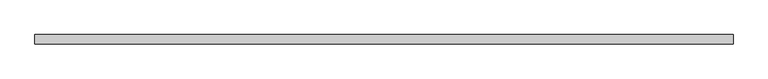
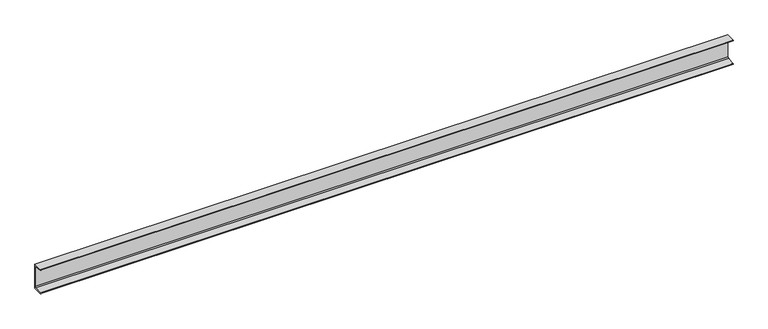
"""IFC4 building model written with IfcOpenShell, lengths in millimetres: beam geometry, C-образный профиль (ГОСТ 8240-89) Балки : [ 22."""

import ifcopenshell
import ifcopenshell.guid

model = None  # the IFC model being written
_history = None  # IfcOwnerHistory: only IFC2X3 demands one
_inside = {}  # id of a spatial element -> (the spatial element, [elements in it])
_under = {}  # id of a project, library or spatial element -> (it, [spatial elements below it])
_declared = {}  # id of a project -> (the project, [libraries it declares])
_typed = {}  # id of a type object -> (the type object, [elements of that type])
_made_of = {}  # id of a material, layer set ... -> (it, [elements and type objects made of it])


def new_model(schema):
    """Start an empty IFC model of exactly this schema.

    Asked for "IFC4X3", IfcOpenShell would pick the latest addendum, in which some entities
    have other attributes; the version numbers below select the first issue.
    IFC2X3 requires an IfcOwnerHistory on every rooted entity: one is made here for all.
    """
    global model, _history
    if schema == "IFC4X3":
        model = ifcopenshell.file(schema_version=(4, 3, 0, 0))
    else:
        model = ifcopenshell.file(schema=schema)
    _inside.clear()
    _under.clear()
    _declared.clear()
    _typed.clear()
    _made_of.clear()
    _history = None
    if model.schema == "IFC2X3":
        org = make("IfcOrganization", Name="unknown")
        user = make(
            "IfcPersonAndOrganization",
            ThePerson=make("IfcPerson", FamilyName="unknown"),
            TheOrganization=org,
        )
        app = make(
            "IfcApplication",
            ApplicationDeveloper=org,
            Version="unknown",
            ApplicationFullName="unknown",
            ApplicationIdentifier="unknown",
        )
        _history = make(
            "IfcOwnerHistory",
            OwningUser=user,
            OwningApplication=app,
            ChangeAction="ADDED",
            CreationDate=0,
        )
    return model


def make(cls, **values):
    """One entity of the class cls with the attributes given. An attribute that is None is left unset."""
    return model.create_entity(
        cls, **{name: value for name, value in values.items() if value is not None}
    )


def rooted(cls, **values):
    """An entity with a GlobalId (a new one), such as an element, a storey or a relation."""
    return make(cls, GlobalId=ifcopenshell.guid.new(), OwnerHistory=_history, **values)


def si_unit(unit_type, name, prefix=None):
    """IfcSIUnit, for example si_unit("LENGTHUNIT", "METRE", prefix="MILLI")."""
    return make("IfcSIUnit", UnitType=unit_type, Prefix=prefix, Name=name)


def assignment(units):
    """IfcUnitAssignment: the units of a project."""
    return None if units is None else make("IfcUnitAssignment", Units=units)


def point(xyz):
    """IfcCartesianPoint."""
    return None if xyz is None else make("IfcCartesianPoint", Coordinates=xyz)


def direction(xyz):
    """IfcDirection."""
    return None if xyz is None else make("IfcDirection", DirectionRatios=xyz)


def frame(location, z_axis=None, x_axis=None):
    """IfcAxis2Placement3D, a coordinate frame: its origin and axes. An axis left out is left unset."""
    return make(
        "IfcAxis2Placement3D",
        Location=point(location),
        Axis=direction(z_axis),
        RefDirection=direction(x_axis),
    )


def frame_2d(location, x_axis=None):
    """IfcAxis2Placement2D, a coordinate frame in the plane: its origin and x axis."""
    return make(
        "IfcAxis2Placement2D", Location=point(location), RefDirection=direction(x_axis)
    )


def origin():
    """The frame at (0, 0, 0) with its axes left unset."""
    return frame((0.0, 0.0, 0.0))


def place(relative_to, where):
    """IfcLocalPlacement: puts the frame where relative to a parent placement (None: the world)."""
    return make(
        "IfcLocalPlacement", PlacementRelTo=relative_to, RelativePlacement=where
    )


def context(
    kind, dimensions, precision=None, world=None, true_north=None, identifier=None
):
    """IfcGeometricRepresentationContext, for example the 3D "Model" context."""
    return make(
        "IfcGeometricRepresentationContext",
        ContextIdentifier=identifier,
        ContextType=kind,
        CoordinateSpaceDimension=dimensions,
        Precision=precision,
        WorldCoordinateSystem=world,
        TrueNorth=true_north,
    )


def project(units=None, contexts=None):
    """IfcProject with its units and contexts."""
    return rooted(
        "IfcProject",
        Name="project",
        RepresentationContexts=contexts,
        UnitsInContext=assignment(units),
    )


def spatial(cls, under=None, at=None, **own):
    """A site, building, storey or space (cls), placed at a placement, below another one or the project."""
    s = rooted(cls, ObjectPlacement=at, **own)
    if under is not None:
        _under.setdefault(under.id(), (under, []))[1].append(s)
    return s


def polyline(points):
    """IfcPolyline through the points."""
    return make("IfcPolyline", Points=[point(p) for p in points])


def circle_curve(where, radius):
    """IfcCircle in the frame where."""
    return make("IfcCircle", Position=where, Radius=radius)


def trimmed(basis, trim1, trim2, sense, master):
    """IfcTrimmedCurve: the piece of a basis curve between two trims."""
    return make(
        "IfcTrimmedCurve",
        BasisCurve=basis,
        Trim1=trim1,
        Trim2=trim2,
        SenseAgreement=sense,
        MasterRepresentation=master,
    )


def segment(curve, same_sense, transition):
    """IfcCompositeCurveSegment."""
    return make(
        "IfcCompositeCurveSegment",
        Transition=transition,
        SameSense=same_sense,
        ParentCurve=curve,
    )


def composite_curve(segments, self_intersect=None):
    """IfcCompositeCurve: segments joined end to end."""
    return make("IfcCompositeCurve", Segments=segments, SelfIntersect=self_intersect)


def outline(outer, holes=None, kind="AREA"):
    """IfcArbitraryClosedProfileDef: a profile drawn as a closed curve; with holes, ...WithVoids."""
    if holes is None:
        return make("IfcArbitraryClosedProfileDef", ProfileType=kind, OuterCurve=outer)
    return make(
        "IfcArbitraryProfileDefWithVoids",
        ProfileType=kind,
        OuterCurve=outer,
        InnerCurves=holes,
    )


def extrude(swept, where, along, depth):
    """IfcExtrudedAreaSolid: the profile swept, set in the frame where, extruded along a direction by depth."""
    return make(
        "IfcExtrudedAreaSolid",
        SweptArea=swept,
        Position=where,
        ExtrudedDirection=direction(along),
        Depth=depth,
    )


def shape(context_of_items, identifier, shape_type, items):
    """IfcShapeRepresentation: the items that make up one representation, for example the "Body"."""
    return make(
        "IfcShapeRepresentation",
        ContextOfItems=context_of_items,
        RepresentationIdentifier=identifier,
        RepresentationType=shape_type,
        Items=items,
    )


def source(mapping_origin, context_of_items, identifier, shape_type, items):
    """IfcRepresentationMap: a shape defined once, which mapped items show again and again."""
    return make(
        "IfcRepresentationMap",
        MappingOrigin=mapping_origin,
        MappedRepresentation=shape(context_of_items, identifier, shape_type, items),
    )


def transform(
    local_origin,
    x_axis=None,
    y_axis=None,
    z_axis=None,
    scale=None,
    scale2=None,
    scale3=None,
    uniform=True,
):
    """IfcCartesianTransformationOperator3D, or its non-uniform kind. x_axis, y_axis, z_axis: its Axis1, 2, 3."""
    if uniform:
        return make(
            "IfcCartesianTransformationOperator3D",
            Axis1=direction(x_axis),
            Axis2=direction(y_axis),
            LocalOrigin=point(local_origin),
            Scale=scale,
            Axis3=direction(z_axis),
        )
    return make(
        "IfcCartesianTransformationOperator3DnonUniform",
        Axis1=direction(x_axis),
        Axis2=direction(y_axis),
        LocalOrigin=point(local_origin),
        Scale=scale,
        Axis3=direction(z_axis),
        Scale2=scale2,
        Scale3=scale3,
    )


def mapped(mapping_source, mapping_target):
    """IfcMappedItem: shows the shape of a source again, moved by a transform."""
    return make(
        "IfcMappedItem", MappingSource=mapping_source, MappingTarget=mapping_target
    )


def made_of(thing, what):
    """Note that an element or type object is made of a material, layer set ...; save() writes the relation."""
    if what is not None:
        _made_of.setdefault(what.id(), (what, []))[1].append(thing)
    return thing


def element(
    cls,
    number,
    at=None,
    inside=None,
    cuts=None,
    type_object=None,
    material=None,
    context=None,
    identifier="Body",
    shape_type=None,
    held_by="IfcProductDefinitionShape",
    body=None,
    shapes=None,
    **own,
):
    """One element of the class cls, such as IfcWall. Its Tag is "e" and its number.

    at: its placement. inside: the storey or other place that contains it. cuts: it is an
    opening in that element (IfcRelVoidsElement). A single representation is given by context,
    identifier, shape_type and body (its items); several are given by shapes. held_by: the class
    of the entity that holds the representations. save() writes the other relations.
    """
    e = rooted(cls, Tag="e%d" % number, ObjectPlacement=at, **own)
    if body is not None:
        shapes = [shape(context, identifier, shape_type, body)]
    if shapes is not None:
        e.Representation = make(held_by, Representations=shapes)
    if inside is not None:
        _inside.setdefault(inside.id(), (inside, []))[1].append(e)
    if cuts is not None:
        rooted(
            "IfcRelVoidsElement", RelatingBuildingElement=cuts, RelatedOpeningElement=e
        )
    if type_object is not None:
        _typed.setdefault(type_object.id(), (type_object, []))[1].append(e)
    return made_of(e, material)


def aggregate(whole, parts):
    """IfcRelAggregates: a whole, such as a stair, and the parts it consists of."""
    return rooted("IfcRelAggregates", RelatingObject=whole, RelatedObjects=parts)


def save(model, path):
    """Write the relations noted so far, then the file.

    IfcRelAggregates (storeys below a building ...), IfcRelContainedInSpatialStructure (elements
    in a storey), IfcRelDefinesByType, IfcRelAssociatesMaterial and IfcRelDeclares: one each for
    every whole, place, type object, material and project.
    """
    for whole, parts in _under.values():
        aggregate(whole, parts)
    for where, things in _inside.values():
        rooted(
            "IfcRelContainedInSpatialStructure",
            RelatedElements=things,
            RelatingStructure=where,
        )
    for kind, things in _typed.values():
        rooted("IfcRelDefinesByType", RelatedObjects=things, RelatingType=kind)
    for what, things in _made_of.values():
        rooted("IfcRelAssociatesMaterial", RelatedObjects=things, RelatingMaterial=what)
    for by, libraries in _declared.values():
        rooted("IfcRelDeclares", RelatingContext=by, RelatedDefinitions=libraries)
    model.write(path)


def beam_8819ffcd(model_context):
    return source(origin(), model_context, "Body", "SweptSolid", [
        extrude(outline(composite_curve([segment(polyline([(22.1, 110.0), (22.1, -110.0), (-59.9, -110.0), (-59.9, -108.9686971)]), True, "CONTINUOUS"), segment(trimmed(circle_curve(frame_2d((-55.9, -108.9686971)), 4.0), [point((-59.9, -108.9686971))], [point((-56.3765809, -104.9971897))], False, "CARTESIAN"), True, "CONTINUOUS"), segment(polyline([(-56.3765809, -104.9971897), (7.8914522, -97.2850257)]), True, "CONTINUOUS"), segment(trimmed(circle_curve(frame_2d((6.7, -87.3562574)), 10.0), [point((7.8914522, -97.2850257))], [point((16.7, -87.3562574))], True, "CARTESIAN"), True, "CONTINUOUS"), segment(polyline([(16.7, -87.3562574), (16.7, 87.3562574)]), True, "CONTINUOUS"), segment(trimmed(circle_curve(frame_2d((6.7, 87.3562574)), 10.0), [point((16.7, 87.3562574))], [point((7.8914522, 97.2850257))], True, "CARTESIAN"), True, "CONTINUOUS"), segment(polyline([(7.8914522, 97.2850257), (-56.3765809, 104.9971897)]), True, "CONTINUOUS"), segment(trimmed(circle_curve(frame_2d((-55.9, 108.9686971)), 4.0), [point((-56.3765809, 104.9971897))], [point((-59.9, 108.9686971))], False, "CARTESIAN"), True, "CONTINUOUS"), segment(polyline([(-59.9, 108.9686971), (-59.9, 110.0), (22.1, 110.0)]), True, "CONTINUOUS")], self_intersect=False)), frame((-3000.0, 0.0, 0.0), z_axis=(1.0, 0.0, 0.0), x_axis=(0.0, 1.0, 0.0)), (0.0, 0.0, 1.0), 6000.0),
    ])


if __name__ == "__main__":
    model = new_model("IFC4")
    model_context = context("Model", 3, world=origin())
    ifc_project = project(units=[si_unit("LENGTHUNIT", "METRE", prefix="MILLI")], contexts=[model_context])
    site = spatial("IfcSite", under=ifc_project)
    building = spatial("IfcBuilding", under=site)
    placement = place(None, origin())
    beam_shape = beam_8819ffcd(model_context)
    element("IfcBeam", 1, ObjectType="C-образный профиль (ГОСТ 8240-89) Балки : [ 22", at=placement, inside=building, context=model_context, shape_type="MappedRepresentation", body=[
        mapped(beam_shape, transform((0.0, 0.0, 0.0), x_axis=(1.0, 0.0, 0.0), y_axis=(0.0, 1.0, 0.0), z_axis=(0.0, 0.0, 1.0))),
    ])
    save(model, "model.ifc")

# Revit data of these elements
# Type "C-образный профиль (ГОСТ 8240-89) Балки : [ 22"
#   tf = 9.5 mm
#   ri = 4 mm
#   ra = 10 mm
#   W = 0.20594
#   Vz = 110 mm
#   Vy = 59.9 mm
#   Vpz = 110 mm
#   Vpy = 22.1 mm
#   Уклон = 0.12
#   Length [instance default] = 1500 mm
#   bf = 82 mm
#   d = 220 mm
#   tw = 5.4 mm
#   A = 0.00267 m²
#   Structural Material [instance default] = Металл - Сталь - 345 МПa
#   Assembly Code = ""
# Element 1 (IfcBeam, "C-образный профиль (ГОСТ 8240-89) Балки : [ 22")
#   Structural Material = C235
#   Materials on its faces: "C235"
# Materials
#   "Металл - Сталь - 345 МПa": class "Металл", colour RGB 247 247 247, transparency 0
#   "C235": class "Не назначено", colour RGB 0 0 0, transparency 0
